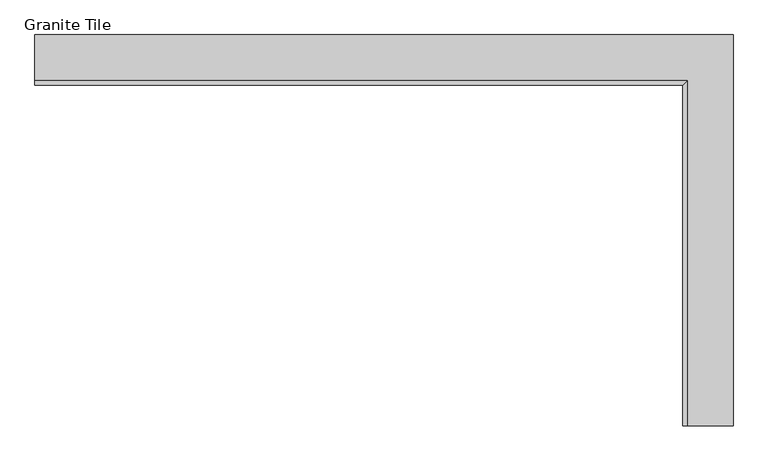
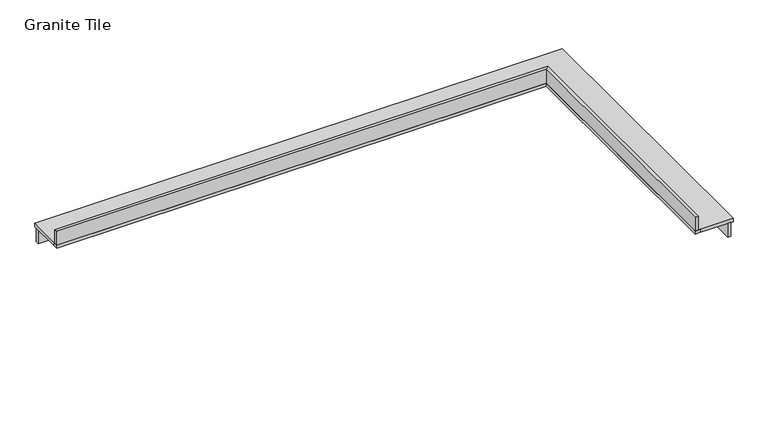
"""IFC4 building model written with IfcOpenShell, lengths in millimetres: stair flight geometry, Granite Tile."""

from ifc_helpers import new_model, si_unit, origin, place, context, project, spatial, faceted_brep, source, transform, mapped, element, save


def granite_tile_49023875(model_context):
    return source(origin(), model_context, "Body", "Brep", [
        faceted_brep([(27480.0, 300.0, 4635.0), (27450.0, 300.0, 4635.0), (27450.0, 300.0, 4500.0), (27480.0, 300.0, 4500.0), (27480.0, 3000.0, 4500.0), (27480.0, 3000.0, 4635.0), (27450.0, 2970.0, 4500.0), (27450.0, 2970.0, 4635.0), (22650.0, 3000.0, 4635.0), (22650.0, 3000.0, 4500.0), (22650.0, 2970.0, 4500.0), (22650.0, 2970.0, 4635.0)], [[[0, 1, 2, 3]], [[4, 5, 0, 3]], [[6, 4, 3, 2]], [[7, 6, 2, 1]], [[5, 7, 1, 0]], [[8, 9, 10, 11]], [[9, 8, 5, 4]], [[10, 9, 4, 6]], [[11, 10, 6, 7]], [[8, 11, 7, 5]]]),
        faceted_brep([(27150.0, 300.0, 4665.0), (27200.0, 300.0, 4665.0), (27500.0, 300.0, 4665.0), (27500.0, 3020.0, 4665.0), (22650.0, 3020.0, 4665.0), (22650.0, 2720.0, 4665.0), (22650.0, 2670.0, 4665.0), (27150.0, 2670.0, 4665.0), (27150.0, 300.0, 4635.0), (27150.0, 2670.0, 4635.0), (22650.0, 2670.0, 4635.0), (22650.0, 2720.0, 4635.0), (22650.0, 3020.0, 4635.0), (27500.0, 3020.0, 4635.0), (27500.0, 300.0, 4635.0), (27200.0, 300.0, 4635.0)], [[[0, 1, 2, 3, 4, 5, 6, 7]], [[8, 9, 10, 11, 12, 13, 14, 15]], [[1, 0, 8, 15]], [[3, 2, 14, 13]], [[5, 4, 12, 11]], [[0, 7, 9, 8]], [[4, 3, 13, 12]], [[7, 6, 10, 9]], [[2, 1, 15, 14]], [[6, 5, 11, 10]]]),
        faceted_brep([(22650.0, 2700.0, 4800.0), (22650.0, 2700.0, 4665.0), (22650.0, 2670.0, 4665.0), (22650.0, 2670.0, 4800.0), (27180.0, 2700.0, 4800.0), (27180.0, 2700.0, 4665.0), (27150.0, 2670.0, 4665.0), (27150.0, 2670.0, 4800.0), (27180.0, 300.0, 4800.0), (27150.0, 300.0, 4800.0), (27150.0, 300.0, 4665.0), (27180.0, 300.0, 4665.0)], [[[0, 1, 2, 3]], [[1, 0, 4, 5]], [[2, 1, 5, 6]], [[3, 2, 6, 7]], [[0, 3, 7, 4]], [[8, 9, 10, 11]], [[5, 4, 8, 11]], [[6, 5, 11, 10]], [[7, 6, 10, 9]], [[4, 7, 9, 8]]]),
    ])


if __name__ == "__main__":
    model = new_model("IFC4")
    model_context = context("Model", 3, world=origin())
    ifc_project = project(units=[si_unit("LENGTHUNIT", "METRE", prefix="MILLI")], contexts=[model_context])
    site = spatial("IfcSite", under=ifc_project)
    building = spatial("IfcBuilding", under=site)
    placement = place(None, origin())
    granite_tile_shape = granite_tile_49023875(model_context)
    element("IfcStairFlight", 1, ObjectType="Granite Tile", at=placement, inside=building, context=model_context, shape_type="MappedRepresentation", body=[
        mapped(granite_tile_shape, transform((0.0, 0.0, 0.0), x_axis=(1.0, 0.0, 0.0), y_axis=(0.0, 1.0, 0.0), z_axis=(0.0, 0.0, 1.0))),
    ])
    save(model, "model.ifc")

# Revit data of these elements
# Element 1 (IfcStairFlight, "Granite Tile")
#   Materials on its faces: "00_Stone_Granite"
# Materials
#   "00_Stone_Granite": class "Stone", colour RGB 99 103 98, transparency 0, Description = "Granite", Cost = 0, Image = Masonry.Stone.Granite.Square.Stacked.Polished.Black-White.jpg
